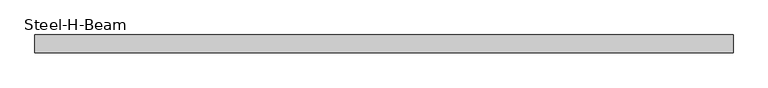
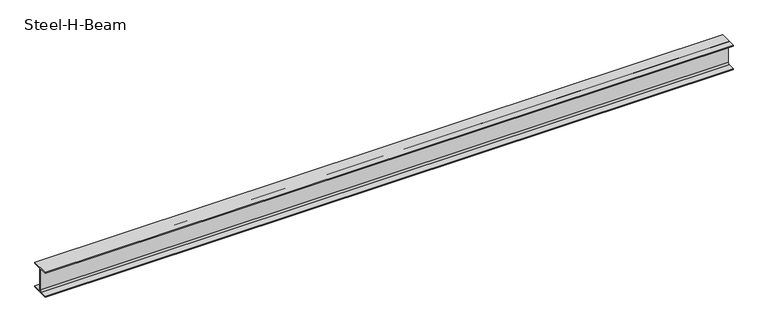
"""IFC4 building model written with IfcOpenShell, lengths in millimetres: beam geometry, Steel-H-Beam : BM121_H-294×200x8x12."""

from ifc_helpers import new_model, si_unit, point, frame, frame_2d, origin, place, context, project, spatial, polyline, circle_curve, trimmed, segment, composite_curve, outline, extrude, source, transform, mapped, element, save


def steel_h_beam_6364cf9a(model_context):
    return source(origin(), model_context, "Body", "SweptSolid", [
        extrude(outline(composite_curve([segment(polyline([(100.0, -135.0), (100.0, -147.0), (-100.0, -147.0), (-100.0, -135.0), (-22.0, -135.0)]), True, "CONTINUOUS"), segment(trimmed(circle_curve(frame_2d((-22.0, -117.0)), 18.0), [point((-22.0, -135.0))], [point((-4.0, -117.0))], True, "CARTESIAN"), True, "CONTINUOUS"), segment(polyline([(-4.0, -117.0), (-4.0, 117.0)]), True, "CONTINUOUS"), segment(trimmed(circle_curve(frame_2d((-22.0, 117.0)), 18.0), [point((-4.0, 117.0))], [point((-22.0, 135.0))], True, "CARTESIAN"), True, "CONTINUOUS"), segment(polyline([(-22.0, 135.0), (-100.0, 135.0), (-100.0, 147.0), (100.0, 147.0), (100.0, 135.0), (22.0, 135.0)]), True, "CONTINUOUS"), segment(trimmed(circle_curve(frame_2d((22.0, 117.0)), 18.0), [point((22.0, 135.0))], [point((4.0, 117.0))], True, "CARTESIAN"), True, "CONTINUOUS"), segment(polyline([(4.0, 117.0), (4.0, -117.0)]), True, "CONTINUOUS"), segment(trimmed(circle_curve(frame_2d((22.0, -117.0)), 18.0), [point((4.0, -117.0))], [point((22.0, -135.0))], True, "CARTESIAN"), True, "CONTINUOUS"), segment(polyline([(22.0, -135.0), (100.0, -135.0)]), True, "CONTINUOUS")], self_intersect=False)), frame((-3880.0, 0.0, 0.0), z_axis=(1.0, 0.0, 0.0), x_axis=(0.0, 1.0, 0.0)), (0.0, 0.0, 1.0), 7760.0),
    ])


if __name__ == "__main__":
    model = new_model("IFC4")
    model_context = context("Model", 3, world=origin())
    ifc_project = project(units=[si_unit("LENGTHUNIT", "METRE", prefix="MILLI")], contexts=[model_context])
    site = spatial("IfcSite", under=ifc_project)
    building = spatial("IfcBuilding", under=site)
    placement = place(None, origin())
    steel_h_beam_shape = steel_h_beam_6364cf9a(model_context)
    element("IfcBeam", 1, ObjectType="Steel-H-Beam : BM121_H-294×200x8x12", at=placement, inside=building, context=model_context, shape_type="MappedRepresentation", body=[
        mapped(steel_h_beam_shape, transform((0.0, 0.0, 0.0), x_axis=(1.0, 0.0, 0.0), y_axis=(0.0, 1.0, 0.0), z_axis=(0.0, 0.0, 1.0))),
    ])
    save(model, "model.ifc")

# Revit data of these elements
# Type "Steel-H-Beam : BM121_H-294×200x8x12"
#   Surface Area = 1.3411 m²/m
#   Section Area = 72.3812 cm²
#   Mass per Unit Length = 56.8193 kg/m
#   Length [instance default] = 3000 mm
#   B = 200 mm
#   H = 294 mm
#   r = 18 mm
#   tw = 8 mm
#   tf = 12 mm
#   hec_material4 [instance default] = none
#   hec_material3 [instance default] = none
#   hec_material2 [instance default] = none
#   hec_material1 [instance default] = none
#   Structural Material [instance default] = Steel, 45-345
#   Assembly Code = ""
# Element 1 (IfcBeam, "Steel-H-Beam : BM121_H-294×200x8x12")
#   hec_material3 = F01AC000-00002_Building/Shelter Fire Proofing Work_Intumescent Coating Type_1 hr. rating (UL 1709))
#   hec_material2 = S01AA010-00002_Main Steel Structure Fabrication Work_Shelter/Building_Steel Painting/Coating_for Fireproofed Steel Surface, Surface Preparation & Primer Coat
#   hec_material1 = S03AA028-00001_Main Steel Structure Erection Work_Shelter/Building_Medium Steel
#   Structural Material = S01AA002-00001_Main Steel Structure Fabrication Work_Shelter/Building_Medium Steel - Standard
#   Materials on its faces: "S01AA002-00001_Main Steel Structure Fabrication Work_Shelter/Building_Medium Steel - Standard"
# Materials
#   "Steel, 45-345": class "Metal", colour RGB 189 187 185, transparency 0, Description = "Steel 345 MPa", Cost = 0
#   "S01AA002-00001_Main Steel Structure Fabrication Work_Shelter/Building_Medium Steel - Standard": class "Metal", colour RGB 120 120 120, transparency 0, Comments = "(90KG/M>Weight≥30KG/M)", Description = "Structural steel 50ksi", W00) Work Master Code = "S01AA002-0001", W01) Work Master_Lv1 = "Main Steel Structure Fabrication Work", W02) Work Master_Lv2 = "Shelter/Building", W03) Work Master_Spec.1 = "Medium Steel - Standard (90KG/M>Weight≥30KG/M)", Cost = 0
#   "F01AC000-00002_Building/Shelter Fire Proofing Work_Intumescent Coating Type_1 hr. rating (UL 1709))": class "Metal", colour RGB 255 128 128, transparency 0, Description = "Paint finished steel", W00) Work Master Code = "F01AC000-00002", W01) Work Master_Lv1 = "Building/Shelter Fire Proofing Work", W02) Work Master_Lv2 = "Intumescent Coating Type", W03) Work Master_Spec.1 = "1 hr. rating (UL 1709)", Cost = 0
#   "S01AA010-00002_Main Steel Structure Fabrication Work_Shelter/Building_Steel Painting/Coating_for Fireproofed Steel Surface, Surface Preparation & Primer Coat": class "Metal", colour RGB 120 120 120, transparency 0, Description = "Paint finished steel", W00) Work Master Code = "SS01AA010-00002", W01) Work Master_Lv1 = "Main Steel Structure Fabrication Work", W02) Work Master_Lv2 = "Shelter/Building", W03) Work Master_Spec.1 = "Steel Painting/Coating", W04) Work Master_Spec.2 = "for Fireproofed Steel Surface, Surface Preparation & Primer Coat", Cost = 0
#   "S03AA028-00001_Main Steel Structure Erection Work_Shelter/Building_Medium Steel": class "Metal", colour RGB 120 120 120, transparency 0, Comments = "(90KG/M>Weight≥30KG/M)", Description = "Structural steel 50ksi", W00) Work Master Code = "S03AA028-0001", W01) Work Master_Lv1 = "Main Steel Structure Erection Work", W02) Work Master_Lv2 = "Shelter/Building", W03) Work Master_Spec.1 = "Medium Steel (90KG/M>Weight≥30KG/M)", Cost = 0
